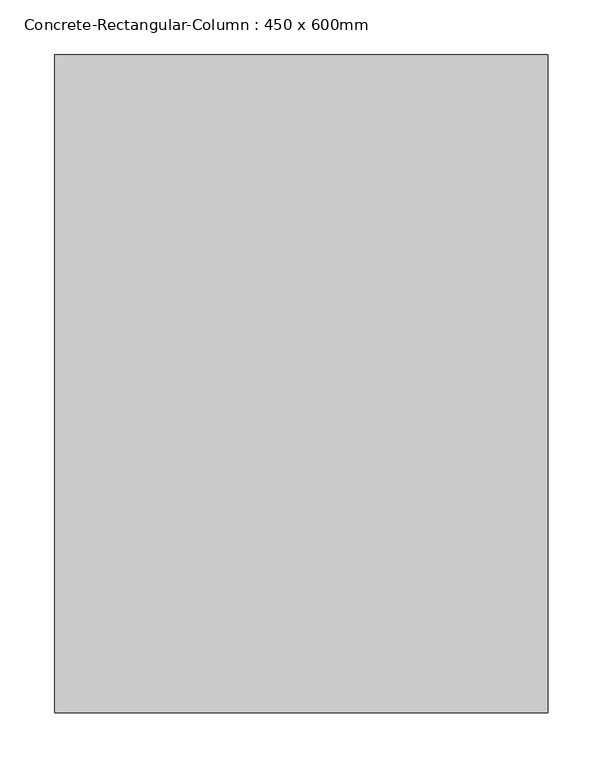
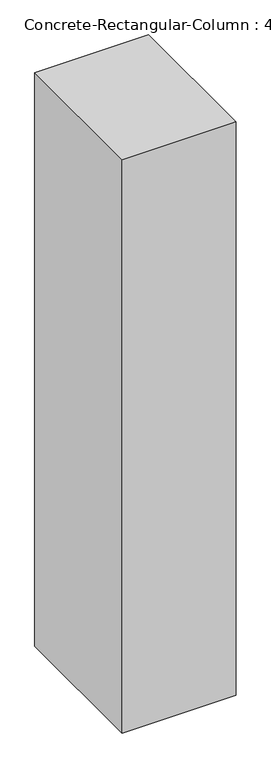
"""IFC4 building model written with IfcOpenShell, lengths in millimetres: column geometry, Concrete-Rectangular-Column : 450 x 600mm."""

from ifc_helpers import new_model, si_unit, frame, origin, place, context, project, spatial, polyline, outline, extrude, source, transform, mapped, element, save


def concrete_rectangular_column_450_x_600mm_14788169(model_context):
    return source(origin(), model_context, "Body", "SweptSolid", [
        extrude(outline(polyline([(225.0, 300.0), (225.0, -300.0), (-225.0, -300.0), (-225.0, 300.0), (225.0, 300.0)])), frame((0.0, 0.0, 3600.0), z_axis=(0.0, 0.0, 1.0), x_axis=(1.0, 0.0, 0.0)), (0.0, 0.0, 1.0), 2400.0),
    ])


if __name__ == "__main__":
    model = new_model("IFC4")
    model_context = context("Model", 3, world=origin())
    ifc_project = project(units=[si_unit("LENGTHUNIT", "METRE", prefix="MILLI")], contexts=[model_context])
    site = spatial("IfcSite", under=ifc_project)
    building = spatial("IfcBuilding", under=site)
    placement = place(None, origin())
    concrete_rectangular_column_450_x_600mm_shape = concrete_rectangular_column_450_x_600mm_14788169(model_context)
    element("IfcColumn", 1, ObjectType="Concrete-Rectangular-Column : 450 x 600mm", at=placement, inside=building, context=model_context, shape_type="MappedRepresentation", body=[
        mapped(concrete_rectangular_column_450_x_600mm_shape, transform((0.0, 0.0, 0.0), x_axis=(1.0, 0.0, 0.0), y_axis=(0.0, 1.0, 0.0), z_axis=(0.0, 0.0, 1.0))),
    ])
    save(model, "model.ifc")

# Revit data of these elements
# Type "Concrete-Rectangular-Column : 450 x 600mm"
#   b = 450 mm
#   h = 600 mm
#   Structural Material [instance default] = Concrete, Cast-in-Place gray
# Element 1 (IfcColumn, "Concrete-Rectangular-Column : 450 x 600mm")
#   Materials on its faces: "Concrete, Cast-in-Place gray"
# Materials
#   "Concrete, Cast-in-Place gray": class "Concrete", colour RGB 192 192 192, transparency 0, Description = "Cast-in-place concrete", Cost = 0
